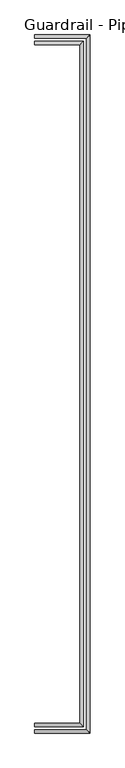
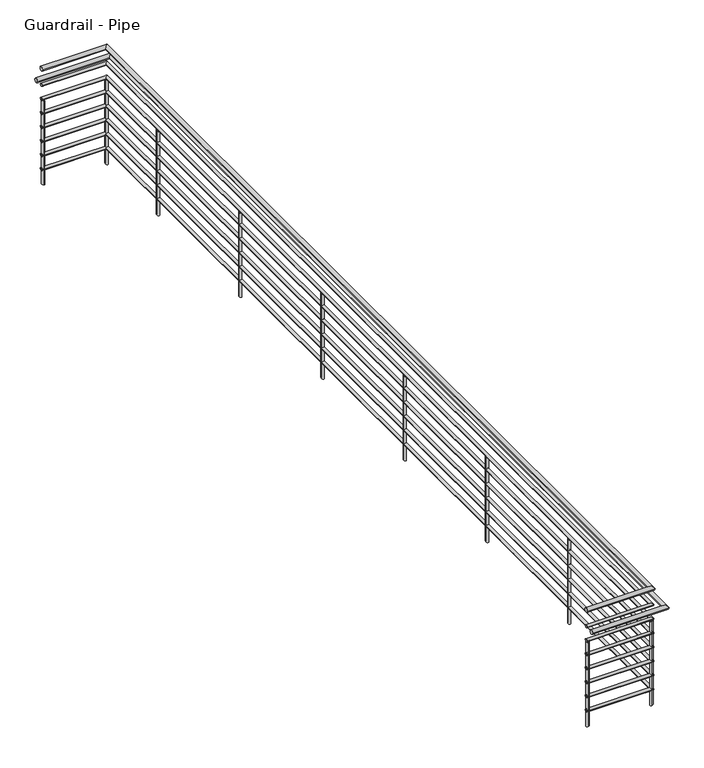
"""IFC4 building model written with IfcOpenShell, lengths in millimetres: railing geometry, Guardrail - Pipe."""

import ifcopenshell
import ifcopenshell.guid

model = None  # the IFC model being written
_history = None  # IfcOwnerHistory: only IFC2X3 demands one
_inside = {}  # id of a spatial element -> (the spatial element, [elements in it])
_under = {}  # id of a project, library or spatial element -> (it, [spatial elements below it])
_declared = {}  # id of a project -> (the project, [libraries it declares])
_typed = {}  # id of a type object -> (the type object, [elements of that type])
_made_of = {}  # id of a material, layer set ... -> (it, [elements and type objects made of it])


def new_model(schema):
    """Start an empty IFC model of exactly this schema.

    Asked for "IFC4X3", IfcOpenShell would pick the latest addendum, in which some entities
    have other attributes; the version numbers below select the first issue.
    IFC2X3 requires an IfcOwnerHistory on every rooted entity: one is made here for all.
    """
    global model, _history
    if schema == "IFC4X3":
        model = ifcopenshell.file(schema_version=(4, 3, 0, 0))
    else:
        model = ifcopenshell.file(schema=schema)
    _inside.clear()
    _under.clear()
    _declared.clear()
    _typed.clear()
    _made_of.clear()
    _history = None
    if model.schema == "IFC2X3":
        org = make("IfcOrganization", Name="unknown")
        user = make(
            "IfcPersonAndOrganization",
            ThePerson=make("IfcPerson", FamilyName="unknown"),
            TheOrganization=org,
        )
        app = make(
            "IfcApplication",
            ApplicationDeveloper=org,
            Version="unknown",
            ApplicationFullName="unknown",
            ApplicationIdentifier="unknown",
        )
        _history = make(
            "IfcOwnerHistory",
            OwningUser=user,
            OwningApplication=app,
            ChangeAction="ADDED",
            CreationDate=0,
        )
    return model


def make(cls, **values):
    """One entity of the class cls with the attributes given. An attribute that is None is left unset."""
    return model.create_entity(
        cls, **{name: value for name, value in values.items() if value is not None}
    )


def rooted(cls, **values):
    """An entity with a GlobalId (a new one), such as an element, a storey or a relation."""
    return make(cls, GlobalId=ifcopenshell.guid.new(), OwnerHistory=_history, **values)


def si_unit(unit_type, name, prefix=None):
    """IfcSIUnit, for example si_unit("LENGTHUNIT", "METRE", prefix="MILLI")."""
    return make("IfcSIUnit", UnitType=unit_type, Prefix=prefix, Name=name)


def assignment(units):
    """IfcUnitAssignment: the units of a project."""
    return None if units is None else make("IfcUnitAssignment", Units=units)


def point(xyz):
    """IfcCartesianPoint."""
    return None if xyz is None else make("IfcCartesianPoint", Coordinates=xyz)


def direction(xyz):
    """IfcDirection."""
    return None if xyz is None else make("IfcDirection", DirectionRatios=xyz)


def frame(location, z_axis=None, x_axis=None):
    """IfcAxis2Placement3D, a coordinate frame: its origin and axes. An axis left out is left unset."""
    return make(
        "IfcAxis2Placement3D",
        Location=point(location),
        Axis=direction(z_axis),
        RefDirection=direction(x_axis),
    )


def origin():
    """The frame at (0, 0, 0) with its axes left unset."""
    return frame((0.0, 0.0, 0.0))


def place(relative_to, where):
    """IfcLocalPlacement: puts the frame where relative to a parent placement (None: the world)."""
    return make(
        "IfcLocalPlacement", PlacementRelTo=relative_to, RelativePlacement=where
    )


def context(
    kind, dimensions, precision=None, world=None, true_north=None, identifier=None
):
    """IfcGeometricRepresentationContext, for example the 3D "Model" context."""
    return make(
        "IfcGeometricRepresentationContext",
        ContextIdentifier=identifier,
        ContextType=kind,
        CoordinateSpaceDimension=dimensions,
        Precision=precision,
        WorldCoordinateSystem=world,
        TrueNorth=true_north,
    )


def project(units=None, contexts=None):
    """IfcProject with its units and contexts."""
    return rooted(
        "IfcProject",
        Name="project",
        RepresentationContexts=contexts,
        UnitsInContext=assignment(units),
    )


def spatial(cls, under=None, at=None, **own):
    """A site, building, storey or space (cls), placed at a placement, below another one or the project."""
    s = rooted(cls, ObjectPlacement=at, **own)
    if under is not None:
        _under.setdefault(under.id(), (under, []))[1].append(s)
    return s


def circle_curve(where, radius):
    """IfcCircle in the frame where."""
    return make("IfcCircle", Position=where, Radius=radius)


def ellipse_curve(where, semi_axis1, semi_axis2):
    """IfcEllipse in the frame where."""
    return make(
        "IfcEllipse", Position=where, SemiAxis1=semi_axis1, SemiAxis2=semi_axis2
    )


def shape(context_of_items, identifier, shape_type, items):
    """IfcShapeRepresentation: the items that make up one representation, for example the "Body"."""
    return make(
        "IfcShapeRepresentation",
        ContextOfItems=context_of_items,
        RepresentationIdentifier=identifier,
        RepresentationType=shape_type,
        Items=items,
    )


def source(mapping_origin, context_of_items, identifier, shape_type, items):
    """IfcRepresentationMap: a shape defined once, which mapped items show again and again."""
    return make(
        "IfcRepresentationMap",
        MappingOrigin=mapping_origin,
        MappedRepresentation=shape(context_of_items, identifier, shape_type, items),
    )


def transform(
    local_origin,
    x_axis=None,
    y_axis=None,
    z_axis=None,
    scale=None,
    scale2=None,
    scale3=None,
    uniform=True,
):
    """IfcCartesianTransformationOperator3D, or its non-uniform kind. x_axis, y_axis, z_axis: its Axis1, 2, 3."""
    if uniform:
        return make(
            "IfcCartesianTransformationOperator3D",
            Axis1=direction(x_axis),
            Axis2=direction(y_axis),
            LocalOrigin=point(local_origin),
            Scale=scale,
            Axis3=direction(z_axis),
        )
    return make(
        "IfcCartesianTransformationOperator3DnonUniform",
        Axis1=direction(x_axis),
        Axis2=direction(y_axis),
        LocalOrigin=point(local_origin),
        Scale=scale,
        Axis3=direction(z_axis),
        Scale2=scale2,
        Scale3=scale3,
    )


def mapped(mapping_source, mapping_target):
    """IfcMappedItem: shows the shape of a source again, moved by a transform."""
    return make(
        "IfcMappedItem", MappingSource=mapping_source, MappingTarget=mapping_target
    )


def made_of(thing, what):
    """Note that an element or type object is made of a material, layer set ...; save() writes the relation."""
    if what is not None:
        _made_of.setdefault(what.id(), (what, []))[1].append(thing)
    return thing


def element(
    cls,
    number,
    at=None,
    inside=None,
    cuts=None,
    type_object=None,
    material=None,
    context=None,
    identifier="Body",
    shape_type=None,
    held_by="IfcProductDefinitionShape",
    body=None,
    shapes=None,
    **own,
):
    """One element of the class cls, such as IfcWall. Its Tag is "e" and its number.

    at: its placement. inside: the storey or other place that contains it. cuts: it is an
    opening in that element (IfcRelVoidsElement). A single representation is given by context,
    identifier, shape_type and body (its items); several are given by shapes. held_by: the class
    of the entity that holds the representations. save() writes the other relations.
    """
    e = rooted(cls, Tag="e%d" % number, ObjectPlacement=at, **own)
    if body is not None:
        shapes = [shape(context, identifier, shape_type, body)]
    if shapes is not None:
        e.Representation = make(held_by, Representations=shapes)
    if inside is not None:
        _inside.setdefault(inside.id(), (inside, []))[1].append(e)
    if cuts is not None:
        rooted(
            "IfcRelVoidsElement", RelatingBuildingElement=cuts, RelatedOpeningElement=e
        )
    if type_object is not None:
        _typed.setdefault(type_object.id(), (type_object, []))[1].append(e)
    return made_of(e, material)


def aggregate(whole, parts):
    """IfcRelAggregates: a whole, such as a stair, and the parts it consists of."""
    return rooted("IfcRelAggregates", RelatingObject=whole, RelatedObjects=parts)


def save(model, path):
    """Write the relations noted so far, then the file.

    IfcRelAggregates (storeys below a building ...), IfcRelContainedInSpatialStructure (elements
    in a storey), IfcRelDefinesByType, IfcRelAssociatesMaterial and IfcRelDeclares: one each for
    every whole, place, type object, material and project.
    """
    for whole, parts in _under.values():
        aggregate(whole, parts)
    for where, things in _inside.values():
        rooted(
            "IfcRelContainedInSpatialStructure",
            RelatedElements=things,
            RelatingStructure=where,
        )
    for kind, things in _typed.values():
        rooted("IfcRelDefinesByType", RelatedObjects=things, RelatingType=kind)
    for what, things in _made_of.values():
        rooted("IfcRelAssociatesMaterial", RelatedObjects=things, RelatingMaterial=what)
    for by, libraries in _declared.values():
        rooted("IfcRelDeclares", RelatingContext=by, RelatedDefinitions=libraries)
    model.write(path)


def plane_surface(at):
    """IfcPlane: the flat surface through the origin of the frame at, square to its z axis."""
    return make("IfcPlane", Position=at)


def cylinder_surface(at, radius):
    """IfcCylindricalSurface: all points at the distance radius from the z axis of the frame at."""
    return make("IfcCylindricalSurface", Position=at, Radius=radius)


def advanced_brep(points, edges, surfaces, faces):
    """IfcAdvancedBrep: a solid bounded by faces that lie on surfaces and meet in shared edges.

    An edge is (start, end): straight between two places in points (the first is 0);
    or (start, end, curve); or (start, end, curve, False) where it runs against its curve.
    A face is (place in surfaces, loops), or (place, loops, False) where it looks against
    its surface's normal. A loop lists edges by number (the first is 1), with a minus sign
    where the edge is run from its end to its start. The first loop is the outer one.
    """
    corners = [point(p) for p in points]
    vertices = [make("IfcVertexPoint", VertexGeometry=c) for c in corners]
    made = []
    for start, end, *more in edges:
        made.append(
            make(
                "IfcEdgeCurve",
                EdgeStart=vertices[start],
                EdgeEnd=vertices[end],
                EdgeGeometry=more[0] if more else make("IfcPolyline", Points=[corners[start], corners[end]]),
                SameSense=more[1] if len(more) > 1 else True,
            )
        )
    hull = []
    for where, loops, *sense in faces:
        bounds = []
        for j, loop in enumerate(loops):
            ring = [make("IfcOrientedEdge", EdgeElement=made[abs(k) - 1], Orientation=k > 0) for k in loop]
            bounds.append(
                make(
                    "IfcFaceOuterBound" if j == 0 else "IfcFaceBound",
                    Bound=make("IfcEdgeLoop", EdgeList=ring),
                    Orientation=True,
                )
            )
        hull.append(make("IfcAdvancedFace", Bounds=bounds, FaceSurface=surfaces[where], SameSense=sense[0] if sense else True))
    return make("IfcAdvancedBrep", Outer=make("IfcClosedShell", CfsFaces=hull))


def guardrail_pipe_35cc9563(model_context):
    return source(origin(), model_context, "Body", "AdvancedBrep", [
        advanced_brep(
        [(13389.3313551, 21840.75, 4705.35), (13389.3313551, 21878.85, 4705.35), (13967.1813551, 21840.75, 4705.35), (13929.0813551, 21878.85, 4705.35), (13967.1813551, 29956.05, 4705.35), (13929.0813551, 29917.95, 4705.35), (13389.3313551, 29956.05, 4705.35), (13389.3313551, 29917.95, 4705.35)],
        [
            (0, 1, circle_curve(frame((13389.3313551, 21859.8, 4705.35), z_axis=(-1.0, 0.0, 0.0), x_axis=(0.0, 1.0, 0.0)), 19.05)),
            (1, 0, circle_curve(frame((13389.3313551, 21859.8, 4705.35), z_axis=(-1.0, 0.0, 0.0), x_axis=(0.0, 1.0, 0.0)), 19.05)),
            (0, 2),
            (2, 3, ellipse_curve(frame((13948.1313551, 21859.8, 4705.35), z_axis=(-0.7071067811865475, -0.7071067811865475, 0.0), x_axis=(-0.7071067811865476, 0.7071067811865474, 0.0)), 26.9407684, 19.05)),
            (3, 1),
            (3, 2, ellipse_curve(frame((13948.1313551, 21859.8, 4705.35), z_axis=(-0.7071067811865475, -0.7071067811865475, 0.0), x_axis=(-0.7071067811865476, 0.7071067811865474, 0.0)), 26.9407684, 19.05)),
            (2, 4),
            (4, 5, ellipse_curve(frame((13948.1313551, 29937.0, 4705.35), z_axis=(0.7071067811865475, -0.7071067811865475, 0.0), x_axis=(-0.7071067811865474, -0.7071067811865476, 0.0)), 26.9407684, 19.05)),
            (5, 3),
            (5, 4, ellipse_curve(frame((13948.1313551, 29937.0, 4705.35), z_axis=(0.7071067811865475, -0.7071067811865475, 0.0), x_axis=(-0.7071067811865474, -0.7071067811865476, 0.0)), 26.9407684, 19.05)),
            (6, 7, circle_curve(frame((13389.3313551, 29937.0, 4705.35), z_axis=(-1.0, 0.0, 0.0), x_axis=(0.0, -1.0, 0.0)), 19.05)),
            (7, 6, circle_curve(frame((13389.3313551, 29937.0, 4705.35), z_axis=(-1.0, 0.0, 0.0), x_axis=(0.0, -1.0, 0.0)), 19.05)),
            (4, 6),
            (7, 5),
        ],
        [
            plane_surface(frame((13389.3313551, 21859.8, 4724.4), z_axis=(-1.0, 0.0, 0.0), x_axis=(0.0, 1.0, 0.0))),
            cylinder_surface(frame((13389.3313551, 21859.8, 4705.35), z_axis=(-1.0, 0.0, 0.0), x_axis=(0.0, 1.0, 0.0)), 19.05),
            cylinder_surface(frame((13948.1313551, 21859.8, 4705.35), z_axis=(0.0, -1.0, 0.0), x_axis=(-1.0, 0.0, 0.0)), 19.05),
            plane_surface(frame((13389.3313551, 29937.0, 4724.4), z_axis=(-1.0, 0.0, 0.0), x_axis=(0.0, -1.0, 0.0))),
            cylinder_surface(frame((13948.1313551, 29937.0, 4705.35), z_axis=(1.0, 0.0, 0.0), x_axis=(0.0, -1.0, 0.0)), 19.05),
        ],
        [
            (0, [[1, 2]]),
            (1, [[-1, 3, 4, 5]]),
            (1, [[-2, -5, 6, -3]]),
            (2, [[-4, 7, 8, 9]]),
            (2, [[-6, -9, 10, -7]]),
            (3, [[11, 12]]),
            (4, [[-8, 13, -12, 14]]),
            (4, [[-10, -14, -11, -13]]),
        ],
    ),
        advanced_brep(
        [(13389.3313551, 21847.1, 4559.3), (13389.3313551, 21872.5, 4559.3), (13960.8313551, 21847.1, 4559.3), (13935.4313551, 21872.5, 4559.3), (13960.8313551, 29949.7, 4559.3), (13935.4313551, 29924.3, 4559.3), (13389.3313551, 29949.7, 4559.3), (13389.3313551, 29924.3, 4559.3)],
        [
            (0, 1, circle_curve(frame((13389.3313551, 21859.8, 4559.3), z_axis=(-1.0, 0.0, 0.0), x_axis=(0.0, 1.0, 0.0)), 12.7)),
            (1, 0, circle_curve(frame((13389.3313551, 21859.8, 4559.3), z_axis=(-1.0, 0.0, 0.0), x_axis=(0.0, 1.0, 0.0)), 12.7)),
            (0, 2),
            (2, 3, ellipse_curve(frame((13948.1313551, 21859.8, 4559.3), z_axis=(-0.7071067811865475, -0.7071067811865475, 0.0), x_axis=(-0.7071067811865476, 0.7071067811865474, 0.0)), 17.9605122, 12.7)),
            (3, 1),
            (3, 2, ellipse_curve(frame((13948.1313551, 21859.8, 4559.3), z_axis=(-0.7071067811865475, -0.7071067811865475, 0.0), x_axis=(-0.7071067811865476, 0.7071067811865474, 0.0)), 17.9605122, 12.7)),
            (2, 4),
            (4, 5, ellipse_curve(frame((13948.1313551, 29937.0, 4559.3), z_axis=(0.7071067811865475, -0.7071067811865475, 0.0), x_axis=(-0.7071067811865474, -0.7071067811865476, 0.0)), 17.9605122, 12.7)),
            (5, 3),
            (5, 4, ellipse_curve(frame((13948.1313551, 29937.0, 4559.3), z_axis=(0.7071067811865475, -0.7071067811865475, 0.0), x_axis=(-0.7071067811865474, -0.7071067811865476, 0.0)), 17.9605122, 12.7)),
            (6, 7, circle_curve(frame((13389.3313551, 29937.0, 4559.3), z_axis=(-1.0, 0.0, 0.0), x_axis=(0.0, -1.0, 0.0)), 12.7)),
            (7, 6, circle_curve(frame((13389.3313551, 29937.0, 4559.3), z_axis=(-1.0, 0.0, 0.0), x_axis=(0.0, -1.0, 0.0)), 12.7)),
            (4, 6),
            (7, 5),
        ],
        [
            plane_surface(frame((13389.3313551, 21859.8, 4572.0), z_axis=(-1.0, 0.0, 0.0), x_axis=(0.0, 1.0, 0.0))),
            cylinder_surface(frame((13389.3313551, 21859.8, 4559.3), z_axis=(-1.0, 0.0, 0.0), x_axis=(0.0, 1.0, 0.0)), 12.7),
            cylinder_surface(frame((13948.1313551, 21859.8, 4559.3), z_axis=(0.0, -1.0, 0.0), x_axis=(-1.0, 0.0, 0.0)), 12.7),
            plane_surface(frame((13389.3313551, 29937.0, 4572.0), z_axis=(-1.0, 0.0, 0.0), x_axis=(0.0, -1.0, 0.0))),
            cylinder_surface(frame((13948.1313551, 29937.0, 4559.3), z_axis=(1.0, 0.0, 0.0), x_axis=(0.0, -1.0, 0.0)), 12.7),
        ],
        [
            (0, [[1, 2]]),
            (1, [[-1, 3, 4, 5]]),
            (1, [[-2, -5, 6, -3]]),
            (2, [[-4, 7, 8, 9]]),
            (2, [[-6, -9, 10, -7]]),
            (3, [[11, 12]]),
            (4, [[-8, 13, -12, 14]]),
            (4, [[-10, -14, -11, -13]]),
        ],
    ),
        advanced_brep(
        [(13389.3313551, 21764.55, 4552.95), (13389.3313551, 21802.65, 4552.95), (14043.3813551, 21764.55, 4552.95), (14005.2813551, 21802.65, 4552.95), (14043.3813551, 30032.25, 4552.95), (14005.2813551, 29994.15, 4552.95), (13389.3313551, 30032.25, 4552.95), (13389.3313551, 29994.15, 4552.95)],
        [
            (0, 1, circle_curve(frame((13389.3313551, 21783.6, 4552.95), z_axis=(-1.0, 0.0, 0.0), x_axis=(0.0, 1.0, 0.0)), 19.05)),
            (1, 0, circle_curve(frame((13389.3313551, 21783.6, 4552.95), z_axis=(-1.0, 0.0, 0.0), x_axis=(0.0, 1.0, 0.0)), 19.05)),
            (0, 2),
            (2, 3, ellipse_curve(frame((14024.3313551, 21783.6, 4552.95), z_axis=(-0.7071067811865475, -0.7071067811865475, 0.0), x_axis=(-0.7071067811865476, 0.7071067811865474, 0.0)), 26.9407684, 19.05)),
            (3, 1),
            (3, 2, ellipse_curve(frame((14024.3313551, 21783.6, 4552.95), z_axis=(-0.7071067811865475, -0.7071067811865475, 0.0), x_axis=(-0.7071067811865476, 0.7071067811865474, 0.0)), 26.9407684, 19.05)),
            (2, 4),
            (4, 5, ellipse_curve(frame((14024.3313551, 30013.2, 4552.95), z_axis=(0.7071067811865475, -0.7071067811865475, 0.0), x_axis=(-0.7071067811865474, -0.7071067811865476, 0.0)), 26.9407684, 19.05)),
            (5, 3),
            (5, 4, ellipse_curve(frame((14024.3313551, 30013.2, 4552.95), z_axis=(0.7071067811865475, -0.7071067811865475, 0.0), x_axis=(-0.7071067811865474, -0.7071067811865476, 0.0)), 26.9407684, 19.05)),
            (6, 7, circle_curve(frame((13389.3313551, 30013.2, 4552.95), z_axis=(-1.0, 0.0, 0.0), x_axis=(0.0, -1.0, 0.0)), 19.05)),
            (7, 6, circle_curve(frame((13389.3313551, 30013.2, 4552.95), z_axis=(-1.0, 0.0, 0.0), x_axis=(0.0, -1.0, 0.0)), 19.05)),
            (4, 6),
            (7, 5),
        ],
        [
            plane_surface(frame((13389.3313551, 21783.6, 4572.0), z_axis=(-1.0, 0.0, 0.0), x_axis=(0.0, 1.0, 0.0))),
            cylinder_surface(frame((13389.3313551, 21783.6, 4552.95), z_axis=(-1.0, 0.0, 0.0), x_axis=(0.0, 1.0, 0.0)), 19.05),
            cylinder_surface(frame((14024.3313551, 21783.6, 4552.95), z_axis=(0.0, -1.0, 0.0), x_axis=(-1.0, 0.0, 0.0)), 19.05),
            plane_surface(frame((13389.3313551, 30013.2, 4572.0), z_axis=(-1.0, 0.0, 0.0), x_axis=(0.0, -1.0, 0.0))),
            cylinder_surface(frame((14024.3313551, 30013.2, 4552.95), z_axis=(1.0, 0.0, 0.0), x_axis=(0.0, -1.0, 0.0)), 19.05),
        ],
        [
            (0, [[1, 2]]),
            (1, [[-1, 3, 4, 5]]),
            (1, [[-2, -5, 6, -3]]),
            (2, [[-4, 7, 8, 9]]),
            (2, [[-6, -9, 10, -7]]),
            (3, [[11, 12]]),
            (4, [[-8, 13, -12, 14]]),
            (4, [[-10, -14, -11, -13]]),
        ],
    ),
        advanced_brep(
        [(13389.3313551, 21847.1, 4432.3), (13389.3313551, 21872.5, 4432.3), (13960.8313551, 21847.1, 4432.3), (13935.4313551, 21872.5, 4432.3), (13960.8313551, 29949.7, 4432.3), (13935.4313551, 29924.3, 4432.3), (13389.3313551, 29949.7, 4432.3), (13389.3313551, 29924.3, 4432.3)],
        [
            (0, 1, circle_curve(frame((13389.3313551, 21859.8, 4432.3), z_axis=(-1.0, 0.0, 0.0), x_axis=(0.0, 1.0, 0.0)), 12.7)),
            (1, 0, circle_curve(frame((13389.3313551, 21859.8, 4432.3), z_axis=(-1.0, 0.0, 0.0), x_axis=(0.0, 1.0, 0.0)), 12.7)),
            (0, 2),
            (2, 3, ellipse_curve(frame((13948.1313551, 21859.8, 4432.3), z_axis=(-0.7071067811865475, -0.7071067811865475, 0.0), x_axis=(-0.7071067811865476, 0.7071067811865474, 0.0)), 17.9605122, 12.7)),
            (3, 1),
            (3, 2, ellipse_curve(frame((13948.1313551, 21859.8, 4432.3), z_axis=(-0.7071067811865475, -0.7071067811865475, 0.0), x_axis=(-0.7071067811865476, 0.7071067811865474, 0.0)), 17.9605122, 12.7)),
            (2, 4),
            (4, 5, ellipse_curve(frame((13948.1313551, 29937.0, 4432.3), z_axis=(0.7071067811865475, -0.7071067811865475, 0.0), x_axis=(-0.7071067811865474, -0.7071067811865476, 0.0)), 17.9605122, 12.7)),
            (5, 3),
            (5, 4, ellipse_curve(frame((13948.1313551, 29937.0, 4432.3), z_axis=(0.7071067811865475, -0.7071067811865475, 0.0), x_axis=(-0.7071067811865474, -0.7071067811865476, 0.0)), 17.9605122, 12.7)),
            (6, 7, circle_curve(frame((13389.3313551, 29937.0, 4432.3), z_axis=(-1.0, 0.0, 0.0), x_axis=(0.0, -1.0, 0.0)), 12.7)),
            (7, 6, circle_curve(frame((13389.3313551, 29937.0, 4432.3), z_axis=(-1.0, 0.0, 0.0), x_axis=(0.0, -1.0, 0.0)), 12.7)),
            (4, 6),
            (7, 5),
        ],
        [
            plane_surface(frame((13389.3313551, 21859.8, 4445.0), z_axis=(-1.0, 0.0, 0.0), x_axis=(0.0, 1.0, 0.0))),
            cylinder_surface(frame((13389.3313551, 21859.8, 4432.3), z_axis=(-1.0, 0.0, 0.0), x_axis=(0.0, 1.0, 0.0)), 12.7),
            cylinder_surface(frame((13948.1313551, 21859.8, 4432.3), z_axis=(0.0, -1.0, 0.0), x_axis=(-1.0, 0.0, 0.0)), 12.7),
            plane_surface(frame((13389.3313551, 29937.0, 4445.0), z_axis=(-1.0, 0.0, 0.0), x_axis=(0.0, -1.0, 0.0))),
            cylinder_surface(frame((13948.1313551, 29937.0, 4432.3), z_axis=(1.0, 0.0, 0.0), x_axis=(0.0, -1.0, 0.0)), 12.7),
        ],
        [
            (0, [[1, 2]]),
            (1, [[-1, 3, 4, 5]]),
            (1, [[-2, -5, 6, -3]]),
            (2, [[-4, 7, 8, 9]]),
            (2, [[-6, -9, 10, -7]]),
            (3, [[11, 12]]),
            (4, [[-8, 13, -12, 14]]),
            (4, [[-10, -14, -11, -13]]),
        ],
    ),
        advanced_brep(
        [(13389.3313551, 21847.1, 4305.3), (13389.3313551, 21872.5, 4305.3), (13960.8313551, 21847.1, 4305.3), (13935.4313551, 21872.5, 4305.3), (13960.8313551, 29949.7, 4305.3), (13935.4313551, 29924.3, 4305.3), (13389.3313551, 29949.7, 4305.3), (13389.3313551, 29924.3, 4305.3)],
        [
            (0, 1, circle_curve(frame((13389.3313551, 21859.8, 4305.3), z_axis=(-1.0, 0.0, 0.0), x_axis=(0.0, 1.0, 0.0)), 12.7)),
            (1, 0, circle_curve(frame((13389.3313551, 21859.8, 4305.3), z_axis=(-1.0, 0.0, 0.0), x_axis=(0.0, 1.0, 0.0)), 12.7)),
            (0, 2),
            (2, 3, ellipse_curve(frame((13948.1313551, 21859.8, 4305.3), z_axis=(-0.7071067811865475, -0.7071067811865475, 0.0), x_axis=(-0.7071067811865476, 0.7071067811865474, 0.0)), 17.9605122, 12.7)),
            (3, 1),
            (3, 2, ellipse_curve(frame((13948.1313551, 21859.8, 4305.3), z_axis=(-0.7071067811865475, -0.7071067811865475, 0.0), x_axis=(-0.7071067811865476, 0.7071067811865474, 0.0)), 17.9605122, 12.7)),
            (2, 4),
            (4, 5, ellipse_curve(frame((13948.1313551, 29937.0, 4305.3), z_axis=(0.7071067811865475, -0.7071067811865475, 0.0), x_axis=(-0.7071067811865474, -0.7071067811865476, 0.0)), 17.9605122, 12.7)),
            (5, 3),
            (5, 4, ellipse_curve(frame((13948.1313551, 29937.0, 4305.3), z_axis=(0.7071067811865475, -0.7071067811865475, 0.0), x_axis=(-0.7071067811865474, -0.7071067811865476, 0.0)), 17.9605122, 12.7)),
            (6, 7, circle_curve(frame((13389.3313551, 29937.0, 4305.3), z_axis=(-1.0, 0.0, 0.0), x_axis=(0.0, -1.0, 0.0)), 12.7)),
            (7, 6, circle_curve(frame((13389.3313551, 29937.0, 4305.3), z_axis=(-1.0, 0.0, 0.0), x_axis=(0.0, -1.0, 0.0)), 12.7)),
            (4, 6),
            (7, 5),
        ],
        [
            plane_surface(frame((13389.3313551, 21859.8, 4318.0), z_axis=(-1.0, 0.0, 0.0), x_axis=(0.0, 1.0, 0.0))),
            cylinder_surface(frame((13389.3313551, 21859.8, 4305.3), z_axis=(-1.0, 0.0, 0.0), x_axis=(0.0, 1.0, 0.0)), 12.7),
            cylinder_surface(frame((13948.1313551, 21859.8, 4305.3), z_axis=(0.0, -1.0, 0.0), x_axis=(-1.0, 0.0, 0.0)), 12.7),
            plane_surface(frame((13389.3313551, 29937.0, 4318.0), z_axis=(-1.0, 0.0, 0.0), x_axis=(0.0, -1.0, 0.0))),
            cylinder_surface(frame((13948.1313551, 29937.0, 4305.3), z_axis=(1.0, 0.0, 0.0), x_axis=(0.0, -1.0, 0.0)), 12.7),
        ],
        [
            (0, [[1, 2]]),
            (1, [[-1, 3, 4, 5]]),
            (1, [[-2, -5, 6, -3]]),
            (2, [[-4, 7, 8, 9]]),
            (2, [[-6, -9, 10, -7]]),
            (3, [[11, 12]]),
            (4, [[-8, 13, -12, 14]]),
            (4, [[-10, -14, -11, -13]]),
        ],
    ),
        advanced_brep(
        [(13389.3313551, 21847.1, 4178.3), (13389.3313551, 21872.5, 4178.3), (13960.8313551, 21847.1, 4178.3), (13935.4313551, 21872.5, 4178.3), (13960.8313551, 29949.7, 4178.3), (13935.4313551, 29924.3, 4178.3), (13389.3313551, 29949.7, 4178.3), (13389.3313551, 29924.3, 4178.3)],
        [
            (0, 1, circle_curve(frame((13389.3313551, 21859.8, 4178.3), z_axis=(-1.0, 0.0, 0.0), x_axis=(0.0, 1.0, 0.0)), 12.7)),
            (1, 0, circle_curve(frame((13389.3313551, 21859.8, 4178.3), z_axis=(-1.0, 0.0, 0.0), x_axis=(0.0, 1.0, 0.0)), 12.7)),
            (0, 2),
            (2, 3, ellipse_curve(frame((13948.1313551, 21859.8, 4178.3), z_axis=(-0.7071067811865475, -0.7071067811865475, 0.0), x_axis=(-0.7071067811865476, 0.7071067811865474, 0.0)), 17.9605122, 12.7)),
            (3, 1),
            (3, 2, ellipse_curve(frame((13948.1313551, 21859.8, 4178.3), z_axis=(-0.7071067811865475, -0.7071067811865475, 0.0), x_axis=(-0.7071067811865476, 0.7071067811865474, 0.0)), 17.9605122, 12.7)),
            (2, 4),
            (4, 5, ellipse_curve(frame((13948.1313551, 29937.0, 4178.3), z_axis=(0.7071067811865475, -0.7071067811865475, 0.0), x_axis=(-0.7071067811865474, -0.7071067811865476, 0.0)), 17.9605122, 12.7)),
            (5, 3),
            (5, 4, ellipse_curve(frame((13948.1313551, 29937.0, 4178.3), z_axis=(0.7071067811865475, -0.7071067811865475, 0.0), x_axis=(-0.7071067811865474, -0.7071067811865476, 0.0)), 17.9605122, 12.7)),
            (6, 7, circle_curve(frame((13389.3313551, 29937.0, 4178.3), z_axis=(-1.0, 0.0, 0.0), x_axis=(0.0, -1.0, 0.0)), 12.7)),
            (7, 6, circle_curve(frame((13389.3313551, 29937.0, 4178.3), z_axis=(-1.0, 0.0, 0.0), x_axis=(0.0, -1.0, 0.0)), 12.7)),
            (4, 6),
            (7, 5),
        ],
        [
            plane_surface(frame((13389.3313551, 21859.8, 4191.0), z_axis=(-1.0, 0.0, 0.0), x_axis=(0.0, 1.0, 0.0))),
            cylinder_surface(frame((13389.3313551, 21859.8, 4178.3), z_axis=(-1.0, 0.0, 0.0), x_axis=(0.0, 1.0, 0.0)), 12.7),
            cylinder_surface(frame((13948.1313551, 21859.8, 4178.3), z_axis=(0.0, -1.0, 0.0), x_axis=(-1.0, 0.0, 0.0)), 12.7),
            plane_surface(frame((13389.3313551, 29937.0, 4191.0), z_axis=(-1.0, 0.0, 0.0), x_axis=(0.0, -1.0, 0.0))),
            cylinder_surface(frame((13948.1313551, 29937.0, 4178.3), z_axis=(1.0, 0.0, 0.0), x_axis=(0.0, -1.0, 0.0)), 12.7),
        ],
        [
            (0, [[1, 2]]),
            (1, [[-1, 3, 4, 5]]),
            (1, [[-2, -5, 6, -3]]),
            (2, [[-4, 7, 8, 9]]),
            (2, [[-6, -9, 10, -7]]),
            (3, [[11, 12]]),
            (4, [[-8, 13, -12, 14]]),
            (4, [[-10, -14, -11, -13]]),
        ],
    ),
        advanced_brep(
        [(13389.3313551, 21847.1, 4051.3), (13389.3313551, 21872.5, 4051.3), (13960.8313551, 21847.1, 4051.3), (13935.4313551, 21872.5, 4051.3), (13960.8313551, 29949.7, 4051.3), (13935.4313551, 29924.3, 4051.3), (13389.3313551, 29949.7, 4051.3), (13389.3313551, 29924.3, 4051.3)],
        [
            (0, 1, circle_curve(frame((13389.3313551, 21859.8, 4051.3), z_axis=(-1.0, 0.0, 0.0), x_axis=(0.0, 1.0, 0.0)), 12.7)),
            (1, 0, circle_curve(frame((13389.3313551, 21859.8, 4051.3), z_axis=(-1.0, 0.0, 0.0), x_axis=(0.0, 1.0, 0.0)), 12.7)),
            (0, 2),
            (2, 3, ellipse_curve(frame((13948.1313551, 21859.8, 4051.3), z_axis=(-0.7071067811865475, -0.7071067811865475, 0.0), x_axis=(-0.7071067811865476, 0.7071067811865474, 0.0)), 17.9605122, 12.7)),
            (3, 1),
            (3, 2, ellipse_curve(frame((13948.1313551, 21859.8, 4051.3), z_axis=(-0.7071067811865475, -0.7071067811865475, 0.0), x_axis=(-0.7071067811865476, 0.7071067811865474, 0.0)), 17.9605122, 12.7)),
            (2, 4),
            (4, 5, ellipse_curve(frame((13948.1313551, 29937.0, 4051.3), z_axis=(0.7071067811865475, -0.7071067811865475, 0.0), x_axis=(-0.7071067811865474, -0.7071067811865476, 0.0)), 17.9605122, 12.7)),
            (5, 3),
            (5, 4, ellipse_curve(frame((13948.1313551, 29937.0, 4051.3), z_axis=(0.7071067811865475, -0.7071067811865475, 0.0), x_axis=(-0.7071067811865474, -0.7071067811865476, 0.0)), 17.9605122, 12.7)),
            (6, 7, circle_curve(frame((13389.3313551, 29937.0, 4051.3), z_axis=(-1.0, 0.0, 0.0), x_axis=(0.0, -1.0, 0.0)), 12.7)),
            (7, 6, circle_curve(frame((13389.3313551, 29937.0, 4051.3), z_axis=(-1.0, 0.0, 0.0), x_axis=(0.0, -1.0, 0.0)), 12.7)),
            (4, 6),
            (7, 5),
        ],
        [
            plane_surface(frame((13389.3313551, 21859.8, 4064.0), z_axis=(-1.0, 0.0, 0.0), x_axis=(0.0, 1.0, 0.0))),
            cylinder_surface(frame((13389.3313551, 21859.8, 4051.3), z_axis=(-1.0, 0.0, 0.0), x_axis=(0.0, 1.0, 0.0)), 12.7),
            cylinder_surface(frame((13948.1313551, 21859.8, 4051.3), z_axis=(0.0, -1.0, 0.0), x_axis=(-1.0, 0.0, 0.0)), 12.7),
            plane_surface(frame((13389.3313551, 29937.0, 4064.0), z_axis=(-1.0, 0.0, 0.0), x_axis=(0.0, -1.0, 0.0))),
            cylinder_surface(frame((13948.1313551, 29937.0, 4051.3), z_axis=(1.0, 0.0, 0.0), x_axis=(0.0, -1.0, 0.0)), 12.7),
        ],
        [
            (0, [[1, 2]]),
            (1, [[-1, 3, 4, 5]]),
            (1, [[-2, -5, 6, -3]]),
            (2, [[-4, 7, 8, 9]]),
            (2, [[-6, -9, 10, -7]]),
            (3, [[11, 12]]),
            (4, [[-8, 13, -12, 14]]),
            (4, [[-10, -14, -11, -13]]),
        ],
    ),
        advanced_brep(
        [(13389.3313551, 21847.1, 3924.3), (13389.3313551, 21872.5, 3924.3), (13960.8313551, 21847.1, 3924.3), (13935.4313551, 21872.5, 3924.3), (13960.8313551, 29949.7, 3924.3), (13935.4313551, 29924.3, 3924.3), (13389.3313551, 29949.7, 3924.3), (13389.3313551, 29924.3, 3924.3)],
        [
            (0, 1, circle_curve(frame((13389.3313551, 21859.8, 3924.3), z_axis=(-1.0, 0.0, 0.0), x_axis=(0.0, 1.0, 0.0)), 12.7)),
            (1, 0, circle_curve(frame((13389.3313551, 21859.8, 3924.3), z_axis=(-1.0, 0.0, 0.0), x_axis=(0.0, 1.0, 0.0)), 12.7)),
            (0, 2),
            (2, 3, ellipse_curve(frame((13948.1313551, 21859.8, 3924.3), z_axis=(-0.7071067811865475, -0.7071067811865475, 0.0), x_axis=(-0.7071067811865476, 0.7071067811865474, 0.0)), 17.9605122, 12.7)),
            (3, 1),
            (3, 2, ellipse_curve(frame((13948.1313551, 21859.8, 3924.3), z_axis=(-0.7071067811865475, -0.7071067811865475, 0.0), x_axis=(-0.7071067811865476, 0.7071067811865474, 0.0)), 17.9605122, 12.7)),
            (2, 4),
            (4, 5, ellipse_curve(frame((13948.1313551, 29937.0, 3924.3), z_axis=(0.7071067811865475, -0.7071067811865475, 0.0), x_axis=(-0.7071067811865474, -0.7071067811865476, 0.0)), 17.9605122, 12.7)),
            (5, 3),
            (5, 4, ellipse_curve(frame((13948.1313551, 29937.0, 3924.3), z_axis=(0.7071067811865475, -0.7071067811865475, 0.0), x_axis=(-0.7071067811865474, -0.7071067811865476, 0.0)), 17.9605122, 12.7)),
            (6, 7, circle_curve(frame((13389.3313551, 29937.0, 3924.3), z_axis=(-1.0, 0.0, 0.0), x_axis=(0.0, -1.0, 0.0)), 12.7)),
            (7, 6, circle_curve(frame((13389.3313551, 29937.0, 3924.3), z_axis=(-1.0, 0.0, 0.0), x_axis=(0.0, -1.0, 0.0)), 12.7)),
            (4, 6),
            (7, 5),
        ],
        [
            plane_surface(frame((13389.3313551, 21859.8, 3937.0), z_axis=(-1.0, 0.0, 0.0), x_axis=(0.0, 1.0, 0.0))),
            cylinder_surface(frame((13389.3313551, 21859.8, 3924.3), z_axis=(-1.0, 0.0, 0.0), x_axis=(0.0, 1.0, 0.0)), 12.7),
            cylinder_surface(frame((13948.1313551, 21859.8, 3924.3), z_axis=(0.0, -1.0, 0.0), x_axis=(-1.0, 0.0, 0.0)), 12.7),
            plane_surface(frame((13389.3313551, 29937.0, 3937.0), z_axis=(-1.0, 0.0, 0.0), x_axis=(0.0, -1.0, 0.0))),
            cylinder_surface(frame((13948.1313551, 29937.0, 3924.3), z_axis=(1.0, 0.0, 0.0), x_axis=(0.0, -1.0, 0.0)), 12.7),
        ],
        [
            (0, [[1, 2]]),
            (1, [[-1, 3, 4, 5]]),
            (1, [[-2, -5, 6, -3]]),
            (2, [[-4, 7, 8, 9]]),
            (2, [[-6, -9, 10, -7]]),
            (3, [[11, 12]]),
            (4, [[-8, 13, -12, 14]]),
            (4, [[-10, -14, -11, -13]]),
        ],
    ),
        advanced_brep(
        [(13389.3313551, 21847.1, 3797.3), (13389.3313551, 21872.5, 3797.3), (13960.8313551, 21847.1, 3797.3), (13935.4313551, 21872.5, 3797.3), (13960.8313551, 29949.7, 3797.3), (13935.4313551, 29924.3, 3797.3), (13389.3313551, 29949.7, 3797.3), (13389.3313551, 29924.3, 3797.3)],
        [
            (0, 1, circle_curve(frame((13389.3313551, 21859.8, 3797.3), z_axis=(-1.0, 0.0, 0.0), x_axis=(0.0, 1.0, 0.0)), 12.7)),
            (1, 0, circle_curve(frame((13389.3313551, 21859.8, 3797.3), z_axis=(-1.0, 0.0, 0.0), x_axis=(0.0, 1.0, 0.0)), 12.7)),
            (0, 2),
            (2, 3, ellipse_curve(frame((13948.1313551, 21859.8, 3797.3), z_axis=(-0.7071067811865475, -0.7071067811865475, 0.0), x_axis=(-0.7071067811865476, 0.7071067811865474, 0.0)), 17.9605122, 12.7)),
            (3, 1),
            (3, 2, ellipse_curve(frame((13948.1313551, 21859.8, 3797.3), z_axis=(-0.7071067811865475, -0.7071067811865475, 0.0), x_axis=(-0.7071067811865476, 0.7071067811865474, 0.0)), 17.9605122, 12.7)),
            (2, 4),
            (4, 5, ellipse_curve(frame((13948.1313551, 29937.0, 3797.3), z_axis=(0.7071067811865475, -0.7071067811865475, 0.0), x_axis=(-0.7071067811865474, -0.7071067811865476, 0.0)), 17.9605122, 12.7)),
            (5, 3),
            (5, 4, ellipse_curve(frame((13948.1313551, 29937.0, 3797.3), z_axis=(0.7071067811865475, -0.7071067811865475, 0.0), x_axis=(-0.7071067811865474, -0.7071067811865476, 0.0)), 17.9605122, 12.7)),
            (6, 7, circle_curve(frame((13389.3313551, 29937.0, 3797.3), z_axis=(-1.0, 0.0, 0.0), x_axis=(0.0, -1.0, 0.0)), 12.7)),
            (7, 6, circle_curve(frame((13389.3313551, 29937.0, 3797.3), z_axis=(-1.0, 0.0, 0.0), x_axis=(0.0, -1.0, 0.0)), 12.7)),
            (4, 6),
            (7, 5),
        ],
        [
            plane_surface(frame((13389.3313551, 21859.8, 3810.0), z_axis=(-1.0, 0.0, 0.0), x_axis=(0.0, 1.0, 0.0))),
            cylinder_surface(frame((13389.3313551, 21859.8, 3797.3), z_axis=(-1.0, 0.0, 0.0), x_axis=(0.0, 1.0, 0.0)), 12.7),
            cylinder_surface(frame((13948.1313551, 21859.8, 3797.3), z_axis=(0.0, -1.0, 0.0), x_axis=(-1.0, 0.0, 0.0)), 12.7),
            plane_surface(frame((13389.3313551, 29937.0, 3810.0), z_axis=(-1.0, 0.0, 0.0), x_axis=(0.0, -1.0, 0.0))),
            cylinder_surface(frame((13948.1313551, 29937.0, 3797.3), z_axis=(1.0, 0.0, 0.0), x_axis=(0.0, -1.0, 0.0)), 12.7),
        ],
        [
            (0, [[1, 2]]),
            (1, [[-1, 3, 4, 5]]),
            (1, [[-2, -5, 6, -3]]),
            (2, [[-4, 7, 8, 9]]),
            (2, [[-6, -9, 10, -7]]),
            (3, [[11, 12]]),
            (4, [[-8, 13, -12, 14]]),
            (4, [[-10, -14, -11, -13]]),
        ],
    ),
        advanced_brep(
        [(13935.4313551, 29175.0, 4419.6), (13960.8313551, 29175.0, 4419.6), (13960.8313551, 29175.0, 3657.6), (13935.4313551, 29175.0, 3657.6)],
        [
            (0, 1, ellipse_curve(frame((13948.1313551, 29175.0, 4419.6), z_axis=(0.0, 0.5368579359867546, -0.8436726596068179), x_axis=(0.0, 0.843672659606818, 0.5368579359867547)), 15.0532317, 12.7)),
            (1, 2),
            (2, 3, ellipse_curve(frame((13948.1313551, 29175.0, 3657.6), z_axis=(0.0, -0.536857935986758, 0.8436726596068158), x_axis=(0.0, 0.8436726596068159, 0.536857935986758)), 15.0532317, 12.7)),
            (3, 0),
            (3, 2, ellipse_curve(frame((13948.1313551, 29175.0, 3657.6), z_axis=(0.0, -0.536857935986758, 0.8436726596068158), x_axis=(0.0, 0.8436726596068159, 0.536857935986758)), 15.0532317, 12.7)),
            (1, 0, ellipse_curve(frame((13948.1313551, 29175.0, 4419.6), z_axis=(0.0, 0.5368579359867546, -0.8436726596068179), x_axis=(0.0, 0.843672659606818, 0.5368579359867547)), 15.0532317, 12.7)),
        ],
        [
            cylinder_surface(frame((13948.1313551, 29175.0, 3429.0), z_axis=(0.0, 0.0, 1.0), x_axis=(1.0, 0.0, 0.0)), 12.7),
            plane_surface(frame((13973.5313551, 29200.4, 4435.7628938), z_axis=(0.0, -0.5368579359867546, 0.8436726596068179), x_axis=(-1.0, 0.0, 0.0))),
            plane_surface(frame((13973.5313551, 29149.6, 3641.4371062), z_axis=(0.0, 0.536857935986758, -0.8436726596068158), x_axis=(-1.0, 0.0, 0.0))),
        ],
        [
            (0, [[1, 2, 3, 4]]),
            (0, [[5, -2, 6, -4]]),
            (1, [[-6, -1]]),
            (2, [[-5, -3]]),
        ],
    ),
        advanced_brep(
        [(13935.4313551, 27955.8, 4419.6), (13960.8313551, 27955.8, 4419.6), (13960.8313551, 27955.8, 3657.6), (13935.4313551, 27955.8, 3657.6)],
        [
            (0, 1, ellipse_curve(frame((13948.1313551, 27955.8, 4419.6), z_axis=(0.0, 0.5368579359867546, -0.8436726596068179), x_axis=(0.0, 0.843672659606818, 0.5368579359867547)), 15.0532317, 12.7)),
            (1, 2),
            (2, 3, ellipse_curve(frame((13948.1313551, 27955.8, 3657.6), z_axis=(0.0, -0.536857935986758, 0.8436726596068158), x_axis=(0.0, 0.8436726596068159, 0.536857935986758)), 15.0532317, 12.7)),
            (3, 0),
            (3, 2, ellipse_curve(frame((13948.1313551, 27955.8, 3657.6), z_axis=(0.0, -0.536857935986758, 0.8436726596068158), x_axis=(0.0, 0.8436726596068159, 0.536857935986758)), 15.0532317, 12.7)),
            (1, 0, ellipse_curve(frame((13948.1313551, 27955.8, 4419.6), z_axis=(0.0, 0.5368579359867546, -0.8436726596068179), x_axis=(0.0, 0.843672659606818, 0.5368579359867547)), 15.0532317, 12.7)),
        ],
        [
            cylinder_surface(frame((13948.1313551, 27955.8, 3429.0), z_axis=(0.0, 0.0, 1.0), x_axis=(1.0, 0.0, 0.0)), 12.7),
            plane_surface(frame((13973.5313551, 27981.2, 4435.7628938), z_axis=(0.0, -0.5368579359867546, 0.8436726596068179), x_axis=(-1.0, 0.0, 0.0))),
            plane_surface(frame((13973.5313551, 27930.4, 3641.4371062), z_axis=(0.0, 0.536857935986758, -0.8436726596068158), x_axis=(-1.0, 0.0, 0.0))),
        ],
        [
            (0, [[1, 2, 3, 4]]),
            (0, [[5, -2, 6, -4]]),
            (1, [[-6, -1]]),
            (2, [[-5, -3]]),
        ],
    ),
        advanced_brep(
        [(13935.4313551, 26736.6, 4419.6), (13960.8313551, 26736.6, 4419.6), (13960.8313551, 26736.6, 3657.6), (13935.4313551, 26736.6, 3657.6)],
        [
            (0, 1, ellipse_curve(frame((13948.1313551, 26736.6, 4419.6), z_axis=(0.0, 0.5368579359867546, -0.8436726596068179), x_axis=(0.0, 0.843672659606818, 0.5368579359867547)), 15.0532317, 12.7)),
            (1, 2),
            (2, 3, ellipse_curve(frame((13948.1313551, 26736.6, 3657.6), z_axis=(0.0, -0.536857935986758, 0.8436726596068158), x_axis=(0.0, 0.8436726596068159, 0.536857935986758)), 15.0532317, 12.7)),
            (3, 0),
            (3, 2, ellipse_curve(frame((13948.1313551, 26736.6, 3657.6), z_axis=(0.0, -0.536857935986758, 0.8436726596068158), x_axis=(0.0, 0.8436726596068159, 0.536857935986758)), 15.0532317, 12.7)),
            (1, 0, ellipse_curve(frame((13948.1313551, 26736.6, 4419.6), z_axis=(0.0, 0.5368579359867546, -0.8436726596068179), x_axis=(0.0, 0.843672659606818, 0.5368579359867547)), 15.0532317, 12.7)),
        ],
        [
            cylinder_surface(frame((13948.1313551, 26736.6, 3429.0), z_axis=(0.0, 0.0, 1.0), x_axis=(1.0, 0.0, 0.0)), 12.7),
            plane_surface(frame((13973.5313551, 26762.0, 4435.7628938), z_axis=(0.0, -0.5368579359867546, 0.8436726596068179), x_axis=(-1.0, 0.0, 0.0))),
            plane_surface(frame((13973.5313551, 26711.2, 3641.4371062), z_axis=(0.0, 0.536857935986758, -0.8436726596068158), x_axis=(-1.0, 0.0, 0.0))),
        ],
        [
            (0, [[1, 2, 3, 4]]),
            (0, [[5, -2, 6, -4]]),
            (1, [[-6, -1]]),
            (2, [[-5, -3]]),
        ],
    ),
        advanced_brep(
        [(13935.4313551, 25517.4, 4419.6), (13960.8313551, 25517.4, 4419.6), (13960.8313551, 25517.4, 3657.6), (13935.4313551, 25517.4, 3657.6)],
        [
            (0, 1, ellipse_curve(frame((13948.1313551, 25517.4, 4419.6), z_axis=(0.0, 0.5368579359867546, -0.8436726596068179), x_axis=(0.0, 0.843672659606818, 0.5368579359867547)), 15.0532317, 12.7)),
            (1, 2),
            (2, 3, ellipse_curve(frame((13948.1313551, 25517.4, 3657.6), z_axis=(0.0, -0.536857935986758, 0.8436726596068158), x_axis=(0.0, 0.8436726596068159, 0.536857935986758)), 15.0532317, 12.7)),
            (3, 0),
            (3, 2, ellipse_curve(frame((13948.1313551, 25517.4, 3657.6), z_axis=(0.0, -0.536857935986758, 0.8436726596068158), x_axis=(0.0, 0.8436726596068159, 0.536857935986758)), 15.0532317, 12.7)),
            (1, 0, ellipse_curve(frame((13948.1313551, 25517.4, 4419.6), z_axis=(0.0, 0.5368579359867546, -0.8436726596068179), x_axis=(0.0, 0.843672659606818, 0.5368579359867547)), 15.0532317, 12.7)),
        ],
        [
            cylinder_surface(frame((13948.1313551, 25517.4, 3429.0), z_axis=(0.0, 0.0, 1.0), x_axis=(1.0, 0.0, 0.0)), 12.7),
            plane_surface(frame((13973.5313551, 25542.8, 4435.7628938), z_axis=(0.0, -0.5368579359867546, 0.8436726596068179), x_axis=(-1.0, 0.0, 0.0))),
            plane_surface(frame((13973.5313551, 25492.0, 3641.4371062), z_axis=(0.0, 0.536857935986758, -0.8436726596068158), x_axis=(-1.0, 0.0, 0.0))),
        ],
        [
            (0, [[1, 2, 3, 4]]),
            (0, [[5, -2, 6, -4]]),
            (1, [[-6, -1]]),
            (2, [[-5, -3]]),
        ],
    ),
        advanced_brep(
        [(13935.4313551, 24298.2, 4419.6), (13960.8313551, 24298.2, 4419.6), (13960.8313551, 24298.2, 3657.6), (13935.4313551, 24298.2, 3657.6)],
        [
            (0, 1, ellipse_curve(frame((13948.1313551, 24298.2, 4419.6), z_axis=(0.0, 0.5368579359867546, -0.8436726596068179), x_axis=(0.0, 0.843672659606818, 0.5368579359867547)), 15.0532317, 12.7)),
            (1, 2),
            (2, 3, ellipse_curve(frame((13948.1313551, 24298.2, 3657.6), z_axis=(0.0, -0.536857935986758, 0.8436726596068158), x_axis=(0.0, 0.8436726596068159, 0.536857935986758)), 15.0532317, 12.7)),
            (3, 0),
            (3, 2, ellipse_curve(frame((13948.1313551, 24298.2, 3657.6), z_axis=(0.0, -0.536857935986758, 0.8436726596068158), x_axis=(0.0, 0.8436726596068159, 0.536857935986758)), 15.0532317, 12.7)),
            (1, 0, ellipse_curve(frame((13948.1313551, 24298.2, 4419.6), z_axis=(0.0, 0.5368579359867546, -0.8436726596068179), x_axis=(0.0, 0.843672659606818, 0.5368579359867547)), 15.0532317, 12.7)),
        ],
        [
            cylinder_surface(frame((13948.1313551, 24298.2, 3429.0), z_axis=(0.0, 0.0, 1.0), x_axis=(1.0, 0.0, 0.0)), 12.7),
            plane_surface(frame((13973.5313551, 24323.6, 4435.7628938), z_axis=(0.0, -0.5368579359867546, 0.8436726596068179), x_axis=(-1.0, 0.0, 0.0))),
            plane_surface(frame((13973.5313551, 24272.8, 3641.4371062), z_axis=(0.0, 0.536857935986758, -0.8436726596068158), x_axis=(-1.0, 0.0, 0.0))),
        ],
        [
            (0, [[1, 2, 3, 4]]),
            (0, [[5, -2, 6, -4]]),
            (1, [[-6, -1]]),
            (2, [[-5, -3]]),
        ],
    ),
        advanced_brep(
        [(13935.4313551, 23079.0, 4419.6), (13960.8313551, 23079.0, 4419.6), (13960.8313551, 23079.0, 3657.6), (13935.4313551, 23079.0, 3657.6)],
        [
            (0, 1, ellipse_curve(frame((13948.1313551, 23079.0, 4419.6), z_axis=(0.0, 0.5368579359867546, -0.8436726596068179), x_axis=(0.0, 0.843672659606818, 0.5368579359867547)), 15.0532317, 12.7)),
            (1, 2),
            (2, 3, ellipse_curve(frame((13948.1313551, 23079.0, 3657.6), z_axis=(0.0, -0.536857935986758, 0.8436726596068158), x_axis=(0.0, 0.8436726596068159, 0.536857935986758)), 15.0532317, 12.7)),
            (3, 0),
            (3, 2, ellipse_curve(frame((13948.1313551, 23079.0, 3657.6), z_axis=(0.0, -0.536857935986758, 0.8436726596068158), x_axis=(0.0, 0.8436726596068159, 0.536857935986758)), 15.0532317, 12.7)),
            (1, 0, ellipse_curve(frame((13948.1313551, 23079.0, 4419.6), z_axis=(0.0, 0.5368579359867546, -0.8436726596068179), x_axis=(0.0, 0.843672659606818, 0.5368579359867547)), 15.0532317, 12.7)),
        ],
        [
            cylinder_surface(frame((13948.1313551, 23079.0, 3429.0), z_axis=(0.0, 0.0, 1.0), x_axis=(1.0, 0.0, 0.0)), 12.7),
            plane_surface(frame((13973.5313551, 23104.4, 4435.7628938), z_axis=(0.0, -0.5368579359867546, 0.8436726596068179), x_axis=(-1.0, 0.0, 0.0))),
            plane_surface(frame((13973.5313551, 23053.6, 3641.4371062), z_axis=(0.0, 0.536857935986758, -0.8436726596068158), x_axis=(-1.0, 0.0, 0.0))),
        ],
        [
            (0, [[1, 2, 3, 4]]),
            (0, [[5, -2, 6, -4]]),
            (1, [[-6, -1]]),
            (2, [[-5, -3]]),
        ],
    ),
        advanced_brep(
        [(13935.4313551, 29937.0, 4419.6), (13960.8313551, 29937.0, 4419.6), (13960.8313551, 29937.0, 3657.6), (13935.4313551, 29937.0, 3657.6)],
        [
            (0, 1, ellipse_curve(frame((13948.1313551, 29937.0, 4419.6), z_axis=(0.0, 0.5368579359867546, -0.8436726596068179), x_axis=(0.0, 0.843672659606818, 0.5368579359867547)), 15.0532317, 12.7)),
            (1, 2),
            (2, 3, ellipse_curve(frame((13948.1313551, 29937.0, 3657.6), z_axis=(0.0, -0.536857935986758, 0.8436726596068158), x_axis=(0.0, 0.8436726596068159, 0.536857935986758)), 15.0532317, 12.7)),
            (3, 0),
            (3, 2, ellipse_curve(frame((13948.1313551, 29937.0, 3657.6), z_axis=(0.0, -0.536857935986758, 0.8436726596068158), x_axis=(0.0, 0.8436726596068159, 0.536857935986758)), 15.0532317, 12.7)),
            (1, 0, ellipse_curve(frame((13948.1313551, 29937.0, 4419.6), z_axis=(0.0, 0.5368579359867546, -0.8436726596068179), x_axis=(0.0, 0.843672659606818, 0.5368579359867547)), 15.0532317, 12.7)),
        ],
        [
            cylinder_surface(frame((13948.1313551, 29937.0, 3429.0), z_axis=(0.0, 0.0, 1.0), x_axis=(1.0, 0.0, 0.0)), 12.7),
            plane_surface(frame((13973.5313551, 29962.4, 4435.7628938), z_axis=(0.0, -0.5368579359867546, 0.8436726596068179), x_axis=(-1.0, 0.0, 0.0))),
            plane_surface(frame((13973.5313551, 29911.6, 3641.4371062), z_axis=(0.0, 0.536857935986758, -0.8436726596068158), x_axis=(-1.0, 0.0, 0.0))),
        ],
        [
            (0, [[1, 2, 3, 4]]),
            (0, [[5, -2, 6, -4]]),
            (1, [[-6, -1]]),
            (2, [[-5, -3]]),
        ],
    ),
        advanced_brep(
        [(13948.1313551, 21872.5, 4419.6), (13948.1313551, 21847.1, 4419.6), (13948.1313551, 21847.1, 3657.6), (13948.1313551, 21872.5, 3657.6)],
        [
            (0, 1, ellipse_curve(frame((13948.1313551, 21859.8, 4419.6), z_axis=(0.5368579359867546, 0.0, -0.8436726596068179), x_axis=(0.843672659606818, 0.0, 0.5368579359867547)), 15.0532317, 12.7)),
            (1, 2),
            (2, 3, ellipse_curve(frame((13948.1313551, 21859.8, 3657.6), z_axis=(-0.536857935986758, 0.0, 0.8436726596068158), x_axis=(0.8436726596068159, 0.0, 0.536857935986758)), 15.0532317, 12.7)),
            (3, 0),
            (3, 2, ellipse_curve(frame((13948.1313551, 21859.8, 3657.6), z_axis=(-0.536857935986758, 0.0, 0.8436726596068158), x_axis=(0.8436726596068159, 0.0, 0.536857935986758)), 15.0532317, 12.7)),
            (1, 0, ellipse_curve(frame((13948.1313551, 21859.8, 4419.6), z_axis=(0.5368579359867546, 0.0, -0.8436726596068179), x_axis=(0.843672659606818, 0.0, 0.5368579359867547)), 15.0532317, 12.7)),
        ],
        [
            cylinder_surface(frame((13948.1313551, 21859.8, 3429.0), z_axis=(0.0, 0.0, 1.0), x_axis=(0.0, -1.0, 0.0)), 12.7),
            plane_surface(frame((13973.5313551, 21834.4, 4435.7628938), z_axis=(-0.5368579359867546, 0.0, 0.8436726596068179), x_axis=(0.0, 1.0, 0.0))),
            plane_surface(frame((13922.7313551, 21834.4, 3641.4371062), z_axis=(0.536857935986758, 0.0, -0.8436726596068158), x_axis=(0.0, 1.0, 0.0))),
        ],
        [
            (0, [[1, 2, 3, 4]]),
            (0, [[5, -2, 6, -4]]),
            (1, [[-6, -1]]),
            (2, [[-5, -3]]),
        ],
    ),
        advanced_brep(
        [(13402.0313551, 29924.3, 4419.6), (13402.0313551, 29949.7, 4419.6), (13402.0313551, 29949.7, 3657.6), (13402.0313551, 29924.3, 3657.6)],
        [
            (0, 1, ellipse_curve(frame((13402.0313551, 29937.0, 4419.6), z_axis=(-0.5368579359867546, 0.0, -0.8436726596068179), x_axis=(-0.843672659606818, 0.0, 0.5368579359867547)), 15.0532317, 12.7)),
            (1, 2),
            (2, 3, ellipse_curve(frame((13402.0313551, 29937.0, 3657.6), z_axis=(0.536857935986758, 0.0, 0.8436726596068158), x_axis=(-0.8436726596068159, 0.0, 0.536857935986758)), 15.0532317, 12.7)),
            (3, 0),
            (3, 2, ellipse_curve(frame((13402.0313551, 29937.0, 3657.6), z_axis=(0.536857935986758, 0.0, 0.8436726596068158), x_axis=(-0.8436726596068159, 0.0, 0.536857935986758)), 15.0532317, 12.7)),
            (1, 0, ellipse_curve(frame((13402.0313551, 29937.0, 4419.6), z_axis=(-0.5368579359867546, 0.0, -0.8436726596068179), x_axis=(-0.843672659606818, 0.0, 0.5368579359867547)), 15.0532317, 12.7)),
        ],
        [
            cylinder_surface(frame((13402.0313551, 29937.0, 3429.0), z_axis=(0.0, 0.0, 1.0), x_axis=(0.0, 1.0, 0.0)), 12.7),
            plane_surface(frame((13376.6313551, 29962.4, 4435.7628938), z_axis=(0.5368579359867546, 0.0, 0.8436726596068179), x_axis=(0.0, -1.0, 0.0))),
            plane_surface(frame((13427.4313551, 29962.4, 3641.4371062), z_axis=(-0.536857935986758, 0.0, -0.8436726596068158), x_axis=(0.0, -1.0, 0.0))),
        ],
        [
            (0, [[1, 2, 3, 4]]),
            (0, [[5, -2, 6, -4]]),
            (1, [[-6, -1]]),
            (2, [[-5, -3]]),
        ],
    ),
        advanced_brep(
        [(13402.0313551, 21872.5, 4419.6), (13402.0313551, 21847.1, 4419.6), (13402.0313551, 21847.1, 3657.6), (13402.0313551, 21872.5, 3657.6)],
        [
            (0, 1, ellipse_curve(frame((13402.0313551, 21859.8, 4419.6), z_axis=(0.5368579359867546, 0.0, -0.8436726596068179), x_axis=(0.843672659606818, 0.0, 0.5368579359867547)), 15.0532317, 12.7)),
            (1, 2),
            (2, 3, ellipse_curve(frame((13402.0313551, 21859.8, 3657.6), z_axis=(-0.536857935986758, 0.0, 0.8436726596068158), x_axis=(0.8436726596068159, 0.0, 0.536857935986758)), 15.0532317, 12.7)),
            (3, 0),
            (3, 2, ellipse_curve(frame((13402.0313551, 21859.8, 3657.6), z_axis=(-0.536857935986758, 0.0, 0.8436726596068158), x_axis=(0.8436726596068159, 0.0, 0.536857935986758)), 15.0532317, 12.7)),
            (1, 0, ellipse_curve(frame((13402.0313551, 21859.8, 4419.6), z_axis=(0.5368579359867546, 0.0, -0.8436726596068179), x_axis=(0.843672659606818, 0.0, 0.5368579359867547)), 15.0532317, 12.7)),
        ],
        [
            cylinder_surface(frame((13402.0313551, 21859.8, 3429.0), z_axis=(0.0, 0.0, 1.0), x_axis=(0.0, -1.0, 0.0)), 12.7),
            plane_surface(frame((13427.4313551, 21834.4, 4435.7628938), z_axis=(-0.5368579359867546, 0.0, 0.8436726596068179), x_axis=(0.0, 1.0, 0.0))),
            plane_surface(frame((13376.6313551, 21834.4, 3641.4371062), z_axis=(0.536857935986758, 0.0, -0.8436726596068158), x_axis=(0.0, 1.0, 0.0))),
        ],
        [
            (0, [[1, 2, 3, 4]]),
            (0, [[5, -2, 6, -4]]),
            (1, [[-6, -1]]),
            (2, [[-5, -3]]),
        ],
    ),
    ])


if __name__ == "__main__":
    model = new_model("IFC4")
    model_context = context("Model", 3, world=origin())
    ifc_project = project(units=[si_unit("LENGTHUNIT", "METRE", prefix="MILLI")], contexts=[model_context])
    site = spatial("IfcSite", under=ifc_project)
    building = spatial("IfcBuilding", under=site)
    placement = place(None, origin())
    guardrail_pipe_shape = guardrail_pipe_35cc9563(model_context)
    element("IfcRailing", 1, ObjectType="Guardrail - Pipe", at=placement, inside=building, context=model_context, shape_type="MappedRepresentation", body=[
        mapped(guardrail_pipe_shape, transform((0.0, 0.0, 0.0), x_axis=(1.0, 0.0, 0.0), y_axis=(0.0, 1.0, 0.0), z_axis=(0.0, 0.0, 1.0))),
    ])
    save(model, "model.ifc")
